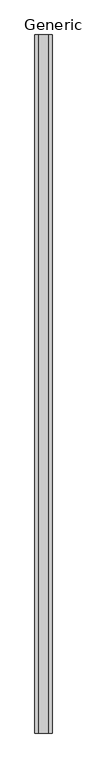
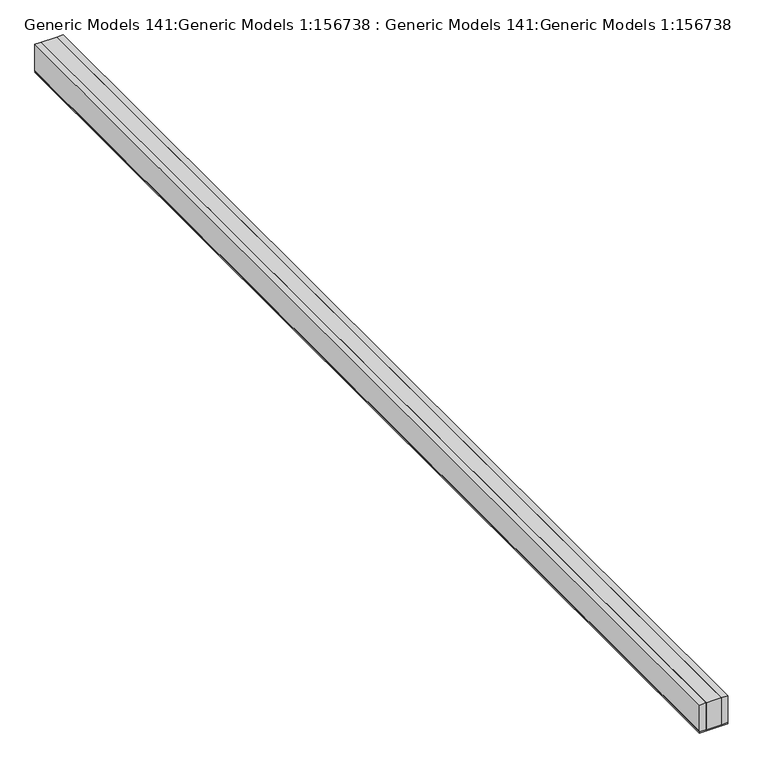
"""IFC4 building model written with IfcOpenShell, lengths in millimetres: proxy geometry, Generic Models 141:Generic Models 1:156738 : Generic Models 141:Generic Models 1:156738."""

import ifcopenshell
import ifcopenshell.guid

model = None  # the IFC model being written
_history = None  # IfcOwnerHistory: only IFC2X3 demands one
_inside = {}  # id of a spatial element -> (the spatial element, [elements in it])
_under = {}  # id of a project, library or spatial element -> (it, [spatial elements below it])
_declared = {}  # id of a project -> (the project, [libraries it declares])
_typed = {}  # id of a type object -> (the type object, [elements of that type])
_made_of = {}  # id of a material, layer set ... -> (it, [elements and type objects made of it])


def new_model(schema):
    """Start an empty IFC model of exactly this schema.

    Asked for "IFC4X3", IfcOpenShell would pick the latest addendum, in which some entities
    have other attributes; the version numbers below select the first issue.
    IFC2X3 requires an IfcOwnerHistory on every rooted entity: one is made here for all.
    """
    global model, _history
    if schema == "IFC4X3":
        model = ifcopenshell.file(schema_version=(4, 3, 0, 0))
    else:
        model = ifcopenshell.file(schema=schema)
    _inside.clear()
    _under.clear()
    _declared.clear()
    _typed.clear()
    _made_of.clear()
    _history = None
    if model.schema == "IFC2X3":
        org = make("IfcOrganization", Name="unknown")
        user = make(
            "IfcPersonAndOrganization",
            ThePerson=make("IfcPerson", FamilyName="unknown"),
            TheOrganization=org,
        )
        app = make(
            "IfcApplication",
            ApplicationDeveloper=org,
            Version="unknown",
            ApplicationFullName="unknown",
            ApplicationIdentifier="unknown",
        )
        _history = make(
            "IfcOwnerHistory",
            OwningUser=user,
            OwningApplication=app,
            ChangeAction="ADDED",
            CreationDate=0,
        )
    return model


def make(cls, **values):
    """One entity of the class cls with the attributes given. An attribute that is None is left unset."""
    return model.create_entity(
        cls, **{name: value for name, value in values.items() if value is not None}
    )


def rooted(cls, **values):
    """An entity with a GlobalId (a new one), such as an element, a storey or a relation."""
    return make(cls, GlobalId=ifcopenshell.guid.new(), OwnerHistory=_history, **values)


def si_unit(unit_type, name, prefix=None):
    """IfcSIUnit, for example si_unit("LENGTHUNIT", "METRE", prefix="MILLI")."""
    return make("IfcSIUnit", UnitType=unit_type, Prefix=prefix, Name=name)


def assignment(units):
    """IfcUnitAssignment: the units of a project."""
    return None if units is None else make("IfcUnitAssignment", Units=units)


def point(xyz):
    """IfcCartesianPoint."""
    return None if xyz is None else make("IfcCartesianPoint", Coordinates=xyz)


def direction(xyz):
    """IfcDirection."""
    return None if xyz is None else make("IfcDirection", DirectionRatios=xyz)


def frame(location, z_axis=None, x_axis=None):
    """IfcAxis2Placement3D, a coordinate frame: its origin and axes. An axis left out is left unset."""
    return make(
        "IfcAxis2Placement3D",
        Location=point(location),
        Axis=direction(z_axis),
        RefDirection=direction(x_axis),
    )


def frame_2d(location, x_axis=None):
    """IfcAxis2Placement2D, a coordinate frame in the plane: its origin and x axis."""
    return make(
        "IfcAxis2Placement2D", Location=point(location), RefDirection=direction(x_axis)
    )


def origin():
    """The frame at (0, 0, 0) with its axes left unset."""
    return frame((0.0, 0.0, 0.0))


def place(relative_to, where):
    """IfcLocalPlacement: puts the frame where relative to a parent placement (None: the world)."""
    return make(
        "IfcLocalPlacement", PlacementRelTo=relative_to, RelativePlacement=where
    )


def context(
    kind, dimensions, precision=None, world=None, true_north=None, identifier=None
):
    """IfcGeometricRepresentationContext, for example the 3D "Model" context."""
    return make(
        "IfcGeometricRepresentationContext",
        ContextIdentifier=identifier,
        ContextType=kind,
        CoordinateSpaceDimension=dimensions,
        Precision=precision,
        WorldCoordinateSystem=world,
        TrueNorth=true_north,
    )


def project(units=None, contexts=None):
    """IfcProject with its units and contexts."""
    return rooted(
        "IfcProject",
        Name="project",
        RepresentationContexts=contexts,
        UnitsInContext=assignment(units),
    )


def spatial(cls, under=None, at=None, **own):
    """A site, building, storey or space (cls), placed at a placement, below another one or the project."""
    s = rooted(cls, ObjectPlacement=at, **own)
    if under is not None:
        _under.setdefault(under.id(), (under, []))[1].append(s)
    return s


def polyline(points):
    """IfcPolyline through the points."""
    return make("IfcPolyline", Points=[point(p) for p in points])


def circle_curve(where, radius):
    """IfcCircle in the frame where."""
    return make("IfcCircle", Position=where, Radius=radius)


def trimmed(basis, trim1, trim2, sense, master):
    """IfcTrimmedCurve: the piece of a basis curve between two trims."""
    return make(
        "IfcTrimmedCurve",
        BasisCurve=basis,
        Trim1=trim1,
        Trim2=trim2,
        SenseAgreement=sense,
        MasterRepresentation=master,
    )


def segment(curve, same_sense, transition):
    """IfcCompositeCurveSegment."""
    return make(
        "IfcCompositeCurveSegment",
        Transition=transition,
        SameSense=same_sense,
        ParentCurve=curve,
    )


def composite_curve(segments, self_intersect=None):
    """IfcCompositeCurve: segments joined end to end."""
    return make("IfcCompositeCurve", Segments=segments, SelfIntersect=self_intersect)


def outline(outer, holes=None, kind="AREA"):
    """IfcArbitraryClosedProfileDef: a profile drawn as a closed curve; with holes, ...WithVoids."""
    if holes is None:
        return make("IfcArbitraryClosedProfileDef", ProfileType=kind, OuterCurve=outer)
    return make(
        "IfcArbitraryProfileDefWithVoids",
        ProfileType=kind,
        OuterCurve=outer,
        InnerCurves=holes,
    )


def extrude(swept, where, along, depth):
    """IfcExtrudedAreaSolid: the profile swept, set in the frame where, extruded along a direction by depth."""
    return make(
        "IfcExtrudedAreaSolid",
        SweptArea=swept,
        Position=where,
        ExtrudedDirection=direction(along),
        Depth=depth,
    )


def shape(context_of_items, identifier, shape_type, items):
    """IfcShapeRepresentation: the items that make up one representation, for example the "Body"."""
    return make(
        "IfcShapeRepresentation",
        ContextOfItems=context_of_items,
        RepresentationIdentifier=identifier,
        RepresentationType=shape_type,
        Items=items,
    )


def source(mapping_origin, context_of_items, identifier, shape_type, items):
    """IfcRepresentationMap: a shape defined once, which mapped items show again and again."""
    return make(
        "IfcRepresentationMap",
        MappingOrigin=mapping_origin,
        MappedRepresentation=shape(context_of_items, identifier, shape_type, items),
    )


def transform(
    local_origin,
    x_axis=None,
    y_axis=None,
    z_axis=None,
    scale=None,
    scale2=None,
    scale3=None,
    uniform=True,
):
    """IfcCartesianTransformationOperator3D, or its non-uniform kind. x_axis, y_axis, z_axis: its Axis1, 2, 3."""
    if uniform:
        return make(
            "IfcCartesianTransformationOperator3D",
            Axis1=direction(x_axis),
            Axis2=direction(y_axis),
            LocalOrigin=point(local_origin),
            Scale=scale,
            Axis3=direction(z_axis),
        )
    return make(
        "IfcCartesianTransformationOperator3DnonUniform",
        Axis1=direction(x_axis),
        Axis2=direction(y_axis),
        LocalOrigin=point(local_origin),
        Scale=scale,
        Axis3=direction(z_axis),
        Scale2=scale2,
        Scale3=scale3,
    )


def mapped(mapping_source, mapping_target):
    """IfcMappedItem: shows the shape of a source again, moved by a transform."""
    return make(
        "IfcMappedItem", MappingSource=mapping_source, MappingTarget=mapping_target
    )


def made_of(thing, what):
    """Note that an element or type object is made of a material, layer set ...; save() writes the relation."""
    if what is not None:
        _made_of.setdefault(what.id(), (what, []))[1].append(thing)
    return thing


def element(
    cls,
    number,
    at=None,
    inside=None,
    cuts=None,
    type_object=None,
    material=None,
    context=None,
    identifier="Body",
    shape_type=None,
    held_by="IfcProductDefinitionShape",
    body=None,
    shapes=None,
    **own,
):
    """One element of the class cls, such as IfcWall. Its Tag is "e" and its number.

    at: its placement. inside: the storey or other place that contains it. cuts: it is an
    opening in that element (IfcRelVoidsElement). A single representation is given by context,
    identifier, shape_type and body (its items); several are given by shapes. held_by: the class
    of the entity that holds the representations. save() writes the other relations.
    """
    e = rooted(cls, Tag="e%d" % number, ObjectPlacement=at, **own)
    if body is not None:
        shapes = [shape(context, identifier, shape_type, body)]
    if shapes is not None:
        e.Representation = make(held_by, Representations=shapes)
    if inside is not None:
        _inside.setdefault(inside.id(), (inside, []))[1].append(e)
    if cuts is not None:
        rooted(
            "IfcRelVoidsElement", RelatingBuildingElement=cuts, RelatedOpeningElement=e
        )
    if type_object is not None:
        _typed.setdefault(type_object.id(), (type_object, []))[1].append(e)
    return made_of(e, material)


def aggregate(whole, parts):
    """IfcRelAggregates: a whole, such as a stair, and the parts it consists of."""
    return rooted("IfcRelAggregates", RelatingObject=whole, RelatedObjects=parts)


def save(model, path):
    """Write the relations noted so far, then the file.

    IfcRelAggregates (storeys below a building ...), IfcRelContainedInSpatialStructure (elements
    in a storey), IfcRelDefinesByType, IfcRelAssociatesMaterial and IfcRelDeclares: one each for
    every whole, place, type object, material and project.
    """
    for whole, parts in _under.values():
        aggregate(whole, parts)
    for where, things in _inside.values():
        rooted(
            "IfcRelContainedInSpatialStructure",
            RelatedElements=things,
            RelatingStructure=where,
        )
    for kind, things in _typed.values():
        rooted("IfcRelDefinesByType", RelatedObjects=things, RelatingType=kind)
    for what, things in _made_of.values():
        rooted("IfcRelAssociatesMaterial", RelatedObjects=things, RelatingMaterial=what)
    for by, libraries in _declared.values():
        rooted("IfcRelDeclares", RelatingContext=by, RelatedDefinitions=libraries)
    model.write(path)


def generic_models_141_generic_models_1_156738_generic_models_1ce9487b(model_context):
    return source(origin(), model_context, "Body", "SweptSolid", [
        extrude(outline(polyline([(-10227.7235063, -5303.1974793), (-10227.7235063, 2583.5025207), (-10123.7422563, 2583.5025207), (-10123.7422563, -5303.1974793), (-10227.7235063, -5303.1974793)])), frame((0.0, 0.0, -738.9225126), z_axis=(0.0, 0.0, 1.0), x_axis=(1.0, 0.0, 0.0)), (0.0, 0.0, 1.0), 193.675),
        extrude(outline(polyline([(-10272.5703813, -5303.1974793), (-10272.5703813, 2583.5025207), (-10228.1203813, 2583.5025207), (-10228.1203813, -5303.1974793), (-10272.5703813, -5303.1974793)])), frame((0.0, 0.0, -738.9225126), z_axis=(0.0, 0.0, 1.0), x_axis=(1.0, 0.0, 0.0)), (0.0, 0.0, 1.0), 193.675),
        extrude(outline(polyline([(-10123.3453813, -5303.1974793), (-10123.3453813, 2583.5025207), (-10078.8953813, 2583.5025207), (-10078.8953813, -5303.1974793), (-10123.3453813, -5303.1974793)])), frame((0.0, 0.0, -738.9225126), z_axis=(0.0, 0.0, 1.0), x_axis=(1.0, 0.0, 0.0)), (0.0, 0.0, 1.0), 193.675),
        extrude(outline(composite_curve([segment(trimmed(circle_curve(frame_2d((-743.8834501, -10074.4804257)), 6.35), [point((-748.4475126, -10078.8953813))], [point((-739.3193876, -10078.8953813))], True, "CARTESIAN"), True, "CONTINUOUS"), segment(polyline([(-739.3193876, -10078.8953813), (-739.3193876, -10272.5703813)]), True, "CONTINUOUS"), segment(trimmed(circle_curve(frame_2d((-743.8834501, -10276.985337)), 6.35), [point((-739.3193876, -10272.5703813))], [point((-748.4475126, -10272.5703813))], True, "CARTESIAN"), True, "CONTINUOUS"), segment(polyline([(-748.4475126, -10272.5703813), (-748.4475126, -10078.8953813)]), True, "CONTINUOUS")], self_intersect=False)), frame((0.0, -5303.1974793, 0.0), z_axis=(0.0, 1.0, 0.0), x_axis=(0.0, 0.0, 1.0)), (0.0, 0.0, 1.0), 7886.7),
    ])


if __name__ == "__main__":
    model = new_model("IFC4")
    model_context = context("Model", 3, world=origin())
    ifc_project = project(units=[si_unit("LENGTHUNIT", "METRE", prefix="MILLI")], contexts=[model_context])
    site = spatial("IfcSite", under=ifc_project)
    building = spatial("IfcBuilding", under=site)
    placement = place(None, origin())
    generic_models_141_generic_models_1_156738_generic_models_shape = generic_models_141_generic_models_1_156738_generic_models_1ce9487b(model_context)
    element("IfcBuildingElementProxy", 1, Name="Generic Models 141:Generic Models 1:156738 : Generic Models 141:Generic Models 1:156738", ObjectType="Generic Models 141:Generic Models 1:156738 : Generic Models 141:Generic Models 1:156738", at=placement, inside=building, context=model_context, shape_type="MappedRepresentation", body=[
        mapped(generic_models_141_generic_models_1_156738_generic_models_shape, transform((0.0, 0.0, 0.0), x_axis=(1.0, 0.0, 0.0), y_axis=(0.0, 1.0, 0.0), z_axis=(0.0, 0.0, 1.0))),
    ])
    save(model, "model.ifc")

# Revit data of these elements
# Type "Generic Models 141:Generic Models 1:156738 : Generic Models 141:Generic Models 1:156738"
#   NameOverride = "Generic Models 141:Generic Models 1:156738"
#   ObjectTypeOverride = "Generic Models 141:Generic Models 1"
#   Reference = "Generic Models 1"
#   Category = "Generic Models"
#   Tag = "156738"
# Element 1 (IfcBuildingElementProxy, "Generic Models 141:Generic Models 1:156738 : Generic Models 141:Generic Models 1:156738")
#   Materials on its faces: "_CONCRETE MASONRY UNITS - FILLED CORE - (SEE STRUCT. DWGS) 44407"
# Materials
#   "_CONCRETE MASONRY UNITS - FILLED CORE - (SEE STRUCT. DWGS) 44407": class "Unassigned", colour RGB 191 191 191, transparency 0
